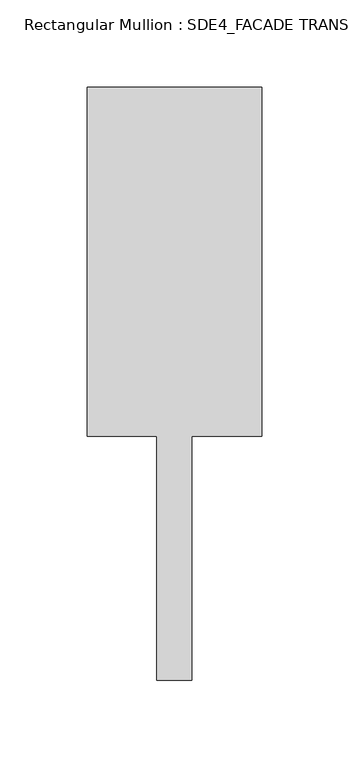
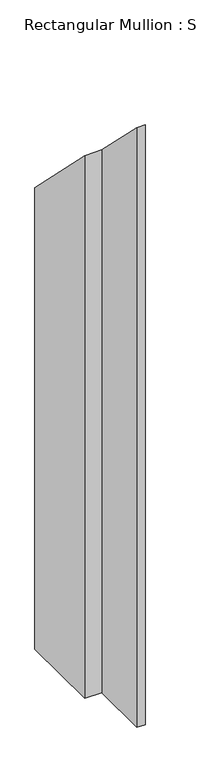
"""IFC4 building model written with IfcOpenShell, lengths in millimetres: member geometry, Rectangular Mullion : SDE4_FACADE TRANSOM TYPE 1."""

from ifc_helpers import new_model, si_unit, origin, place, context, project, spatial, faceted_brep, source, transform, mapped, element, save


def rectangular_mullion_sde4_facade_transom_type_1_6c2b79ce(model_context):
    return source(origin(), model_context, "Body", "Brep", [
        faceted_brep([(50.0, 132.5, -1264.0), (50.0, -67.5, -1264.0), (10.0, -67.5, -1264.0), (10.0, -207.5, -1264.0), (-10.0, -207.5, -1264.0), (-10.0, -67.5, -1264.0), (-50.0, -67.5, -1264.0), (-50.0, 132.5, -1264.0), (-50.0, 132.5, -132.5), (50.0, 132.5, -132.5), (-50.0, -67.5, 67.5), (-10.0, -67.5, 67.5), (-10.0, -207.5, 207.5), (10.0, -207.5, 207.5), (10.0, -67.5, 67.5), (50.0, -67.5, 67.5)], [[[0, 1, 2, 3, 4, 5, 6, 7]], [[8, 9, 0, 7]], [[10, 8, 7, 6]], [[11, 10, 6, 5]], [[12, 11, 5, 4]], [[13, 12, 4, 3]], [[14, 13, 3, 2]], [[15, 14, 2, 1]], [[9, 15, 1, 0]], [[9, 8, 10, 11, 12, 13, 14, 15]]]),
    ])


if __name__ == "__main__":
    model = new_model("IFC4")
    model_context = context("Model", 3, world=origin())
    ifc_project = project(units=[si_unit("LENGTHUNIT", "METRE", prefix="MILLI")], contexts=[model_context])
    site = spatial("IfcSite", under=ifc_project)
    building = spatial("IfcBuilding", under=site)
    placement = place(None, origin())
    rectangular_mullion_sde4_facade_transom_type_1_shape = rectangular_mullion_sde4_facade_transom_type_1_6c2b79ce(model_context)
    element("IfcMember", 1, ObjectType="Rectangular Mullion : SDE4_FACADE TRANSOM TYPE 1", at=placement, inside=building, context=model_context, shape_type="MappedRepresentation", body=[
        mapped(rectangular_mullion_sde4_facade_transom_type_1_shape, transform((0.0, 0.0, 0.0), x_axis=(1.0, 0.0, 0.0), y_axis=(0.0, 1.0, 0.0), z_axis=(0.0, 0.0, 1.0))),
    ])
    save(model, "model.ifc")

# Revit data of these elements
# Type "Rectangular Mullion : SDE4_FACADE TRANSOM TYPE 1"
#   built-in parameter 1007322 = 1.11549 (stored number, unit not read)
#   built-in parameter 1007321 = 0.164042 (stored number, unit not read)
#   built-in parameter 1007320 = 0.164042 (stored number, unit not read)
